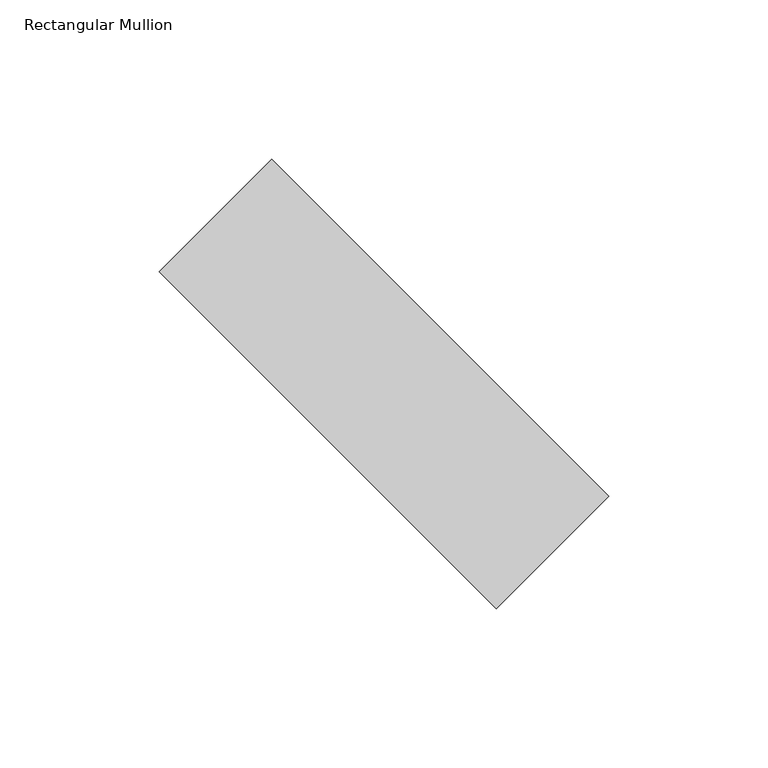
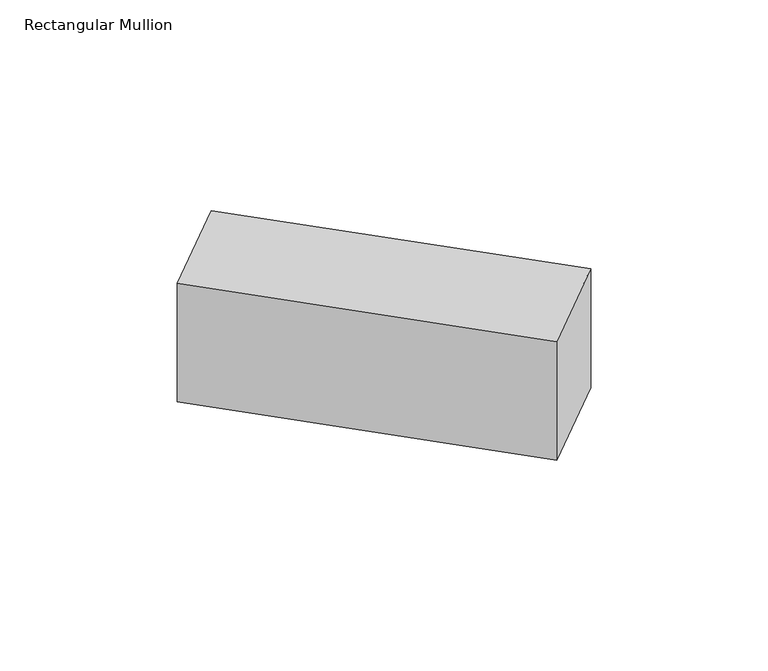
"""IFC4 building model written with IfcOpenShell, lengths in millimetres: member geometry, Rectangular Mullion : tilted mullions."""

import ifcopenshell
import ifcopenshell.guid

model = None  # the IFC model being written
_history = None  # IfcOwnerHistory: only IFC2X3 demands one
_inside = {}  # id of a spatial element -> (the spatial element, [elements in it])
_under = {}  # id of a project, library or spatial element -> (it, [spatial elements below it])
_declared = {}  # id of a project -> (the project, [libraries it declares])
_typed = {}  # id of a type object -> (the type object, [elements of that type])
_made_of = {}  # id of a material, layer set ... -> (it, [elements and type objects made of it])


def new_model(schema):
    """Start an empty IFC model of exactly this schema.

    Asked for "IFC4X3", IfcOpenShell would pick the latest addendum, in which some entities
    have other attributes; the version numbers below select the first issue.
    IFC2X3 requires an IfcOwnerHistory on every rooted entity: one is made here for all.
    """
    global model, _history
    if schema == "IFC4X3":
        model = ifcopenshell.file(schema_version=(4, 3, 0, 0))
    else:
        model = ifcopenshell.file(schema=schema)
    _inside.clear()
    _under.clear()
    _declared.clear()
    _typed.clear()
    _made_of.clear()
    _history = None
    if model.schema == "IFC2X3":
        org = make("IfcOrganization", Name="unknown")
        user = make(
            "IfcPersonAndOrganization",
            ThePerson=make("IfcPerson", FamilyName="unknown"),
            TheOrganization=org,
        )
        app = make(
            "IfcApplication",
            ApplicationDeveloper=org,
            Version="unknown",
            ApplicationFullName="unknown",
            ApplicationIdentifier="unknown",
        )
        _history = make(
            "IfcOwnerHistory",
            OwningUser=user,
            OwningApplication=app,
            ChangeAction="ADDED",
            CreationDate=0,
        )
    return model


def make(cls, **values):
    """One entity of the class cls with the attributes given. An attribute that is None is left unset."""
    return model.create_entity(
        cls, **{name: value for name, value in values.items() if value is not None}
    )


def rooted(cls, **values):
    """An entity with a GlobalId (a new one), such as an element, a storey or a relation."""
    return make(cls, GlobalId=ifcopenshell.guid.new(), OwnerHistory=_history, **values)


def si_unit(unit_type, name, prefix=None):
    """IfcSIUnit, for example si_unit("LENGTHUNIT", "METRE", prefix="MILLI")."""
    return make("IfcSIUnit", UnitType=unit_type, Prefix=prefix, Name=name)


def assignment(units):
    """IfcUnitAssignment: the units of a project."""
    return None if units is None else make("IfcUnitAssignment", Units=units)


def point(xyz):
    """IfcCartesianPoint."""
    return None if xyz is None else make("IfcCartesianPoint", Coordinates=xyz)


def direction(xyz):
    """IfcDirection."""
    return None if xyz is None else make("IfcDirection", DirectionRatios=xyz)


def frame(location, z_axis=None, x_axis=None):
    """IfcAxis2Placement3D, a coordinate frame: its origin and axes. An axis left out is left unset."""
    return make(
        "IfcAxis2Placement3D",
        Location=point(location),
        Axis=direction(z_axis),
        RefDirection=direction(x_axis),
    )


def origin():
    """The frame at (0, 0, 0) with its axes left unset."""
    return frame((0.0, 0.0, 0.0))


def place(relative_to, where):
    """IfcLocalPlacement: puts the frame where relative to a parent placement (None: the world)."""
    return make(
        "IfcLocalPlacement", PlacementRelTo=relative_to, RelativePlacement=where
    )


def context(
    kind, dimensions, precision=None, world=None, true_north=None, identifier=None
):
    """IfcGeometricRepresentationContext, for example the 3D "Model" context."""
    return make(
        "IfcGeometricRepresentationContext",
        ContextIdentifier=identifier,
        ContextType=kind,
        CoordinateSpaceDimension=dimensions,
        Precision=precision,
        WorldCoordinateSystem=world,
        TrueNorth=true_north,
    )


def project(units=None, contexts=None):
    """IfcProject with its units and contexts."""
    return rooted(
        "IfcProject",
        Name="project",
        RepresentationContexts=contexts,
        UnitsInContext=assignment(units),
    )


def spatial(cls, under=None, at=None, **own):
    """A site, building, storey or space (cls), placed at a placement, below another one or the project."""
    s = rooted(cls, ObjectPlacement=at, **own)
    if under is not None:
        _under.setdefault(under.id(), (under, []))[1].append(s)
    return s


def polyline(points):
    """IfcPolyline through the points."""
    return make("IfcPolyline", Points=[point(p) for p in points])


def outline(outer, holes=None, kind="AREA"):
    """IfcArbitraryClosedProfileDef: a profile drawn as a closed curve; with holes, ...WithVoids."""
    if holes is None:
        return make("IfcArbitraryClosedProfileDef", ProfileType=kind, OuterCurve=outer)
    return make(
        "IfcArbitraryProfileDefWithVoids",
        ProfileType=kind,
        OuterCurve=outer,
        InnerCurves=holes,
    )


def extrude(swept, where, along, depth):
    """IfcExtrudedAreaSolid: the profile swept, set in the frame where, extruded along a direction by depth."""
    return make(
        "IfcExtrudedAreaSolid",
        SweptArea=swept,
        Position=where,
        ExtrudedDirection=direction(along),
        Depth=depth,
    )


def shape(context_of_items, identifier, shape_type, items):
    """IfcShapeRepresentation: the items that make up one representation, for example the "Body"."""
    return make(
        "IfcShapeRepresentation",
        ContextOfItems=context_of_items,
        RepresentationIdentifier=identifier,
        RepresentationType=shape_type,
        Items=items,
    )


def source(mapping_origin, context_of_items, identifier, shape_type, items):
    """IfcRepresentationMap: a shape defined once, which mapped items show again and again."""
    return make(
        "IfcRepresentationMap",
        MappingOrigin=mapping_origin,
        MappedRepresentation=shape(context_of_items, identifier, shape_type, items),
    )


def transform(
    local_origin,
    x_axis=None,
    y_axis=None,
    z_axis=None,
    scale=None,
    scale2=None,
    scale3=None,
    uniform=True,
):
    """IfcCartesianTransformationOperator3D, or its non-uniform kind. x_axis, y_axis, z_axis: its Axis1, 2, 3."""
    if uniform:
        return make(
            "IfcCartesianTransformationOperator3D",
            Axis1=direction(x_axis),
            Axis2=direction(y_axis),
            LocalOrigin=point(local_origin),
            Scale=scale,
            Axis3=direction(z_axis),
        )
    return make(
        "IfcCartesianTransformationOperator3DnonUniform",
        Axis1=direction(x_axis),
        Axis2=direction(y_axis),
        LocalOrigin=point(local_origin),
        Scale=scale,
        Axis3=direction(z_axis),
        Scale2=scale2,
        Scale3=scale3,
    )


def mapped(mapping_source, mapping_target):
    """IfcMappedItem: shows the shape of a source again, moved by a transform."""
    return make(
        "IfcMappedItem", MappingSource=mapping_source, MappingTarget=mapping_target
    )


def made_of(thing, what):
    """Note that an element or type object is made of a material, layer set ...; save() writes the relation."""
    if what is not None:
        _made_of.setdefault(what.id(), (what, []))[1].append(thing)
    return thing


def element(
    cls,
    number,
    at=None,
    inside=None,
    cuts=None,
    type_object=None,
    material=None,
    context=None,
    identifier="Body",
    shape_type=None,
    held_by="IfcProductDefinitionShape",
    body=None,
    shapes=None,
    **own,
):
    """One element of the class cls, such as IfcWall. Its Tag is "e" and its number.

    at: its placement. inside: the storey or other place that contains it. cuts: it is an
    opening in that element (IfcRelVoidsElement). A single representation is given by context,
    identifier, shape_type and body (its items); several are given by shapes. held_by: the class
    of the entity that holds the representations. save() writes the other relations.
    """
    e = rooted(cls, Tag="e%d" % number, ObjectPlacement=at, **own)
    if body is not None:
        shapes = [shape(context, identifier, shape_type, body)]
    if shapes is not None:
        e.Representation = make(held_by, Representations=shapes)
    if inside is not None:
        _inside.setdefault(inside.id(), (inside, []))[1].append(e)
    if cuts is not None:
        rooted(
            "IfcRelVoidsElement", RelatingBuildingElement=cuts, RelatedOpeningElement=e
        )
    if type_object is not None:
        _typed.setdefault(type_object.id(), (type_object, []))[1].append(e)
    return made_of(e, material)


def aggregate(whole, parts):
    """IfcRelAggregates: a whole, such as a stair, and the parts it consists of."""
    return rooted("IfcRelAggregates", RelatingObject=whole, RelatedObjects=parts)


def save(model, path):
    """Write the relations noted so far, then the file.

    IfcRelAggregates (storeys below a building ...), IfcRelContainedInSpatialStructure (elements
    in a storey), IfcRelDefinesByType, IfcRelAssociatesMaterial and IfcRelDeclares: one each for
    every whole, place, type object, material and project.
    """
    for whole, parts in _under.values():
        aggregate(whole, parts)
    for where, things in _inside.values():
        rooted(
            "IfcRelContainedInSpatialStructure",
            RelatedElements=things,
            RelatingStructure=where,
        )
    for kind, things in _typed.values():
        rooted("IfcRelDefinesByType", RelatedObjects=things, RelatingType=kind)
    for what, things in _made_of.values():
        rooted("IfcRelAssociatesMaterial", RelatedObjects=things, RelatingMaterial=what)
    for by, libraries in _declared.values():
        rooted("IfcRelDeclares", RelatingContext=by, RelatedDefinitions=libraries)
    model.write(path)


def rectangular_mullion_ce6685f0(model_context):
    return source(origin(), model_context, "Body", "SweptSolid", [
        extrude(outline(polyline([(-35.3553391, 70.7106781), (70.7106781, -35.3553391), (35.3553391, -70.7106781), (-70.7106781, 35.3553391), (-35.3553391, 70.7106781)])), frame((0.0, 0.0, -55.2367034), z_axis=(0.0, 0.0, 1.0), x_axis=(1.0, 0.0, 0.0)), (0.0, 0.0, 1.0), 55.2367034),
    ])


if __name__ == "__main__":
    model = new_model("IFC4")
    model_context = context("Model", 3, world=origin())
    ifc_project = project(units=[si_unit("LENGTHUNIT", "METRE", prefix="MILLI")], contexts=[model_context])
    site = spatial("IfcSite", under=ifc_project)
    building = spatial("IfcBuilding", under=site)
    placement = place(None, origin())
    rectangular_mullion_shape = rectangular_mullion_ce6685f0(model_context)
    element("IfcMember", 1, ObjectType="Rectangular Mullion : tilted mullions", at=placement, inside=building, context=model_context, shape_type="MappedRepresentation", body=[
        mapped(rectangular_mullion_shape, transform((0.0, 0.0, 0.0), x_axis=(1.0, 0.0, 0.0), y_axis=(0.0, 1.0, 0.0), z_axis=(0.0, 0.0, 1.0))),
    ])
    save(model, "model.ifc")

# Revit data of these elements
# Type "Rectangular Mullion : tilted mullions"
#   built-in parameter 1007304 = 0.492126 (stored number, unit not read)
#   built-in parameter 1007301 = 0.082021 (stored number, unit not read)
#   built-in parameter 1007300 = 0.082021 (stored number, unit not read)
# Element 1 (IfcMember, "Rectangular Mullion : tilted mullions")
#   Materials on its faces: "Aluminum"
# Materials
#   "Aluminum": class "Metal", colour RGB 244 244 244, transparency 0, Description = "Aluminum 6061", Cost = 0
